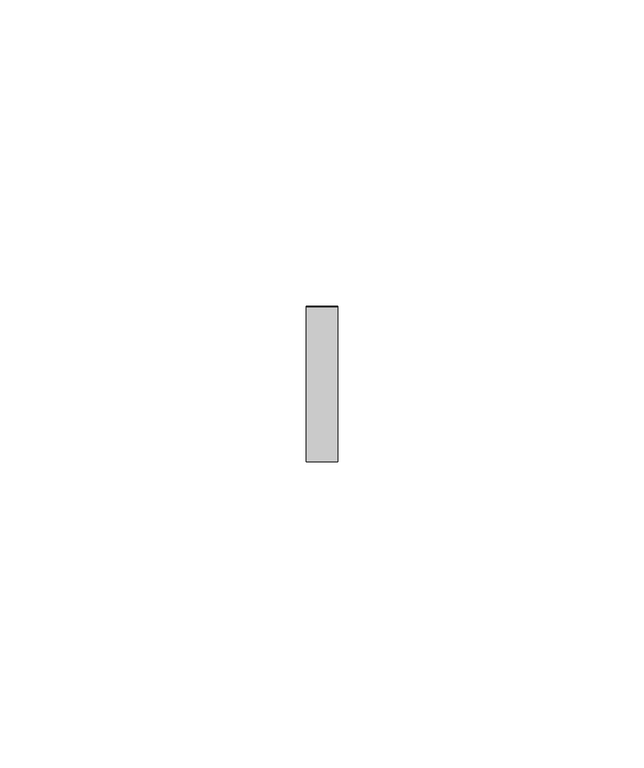
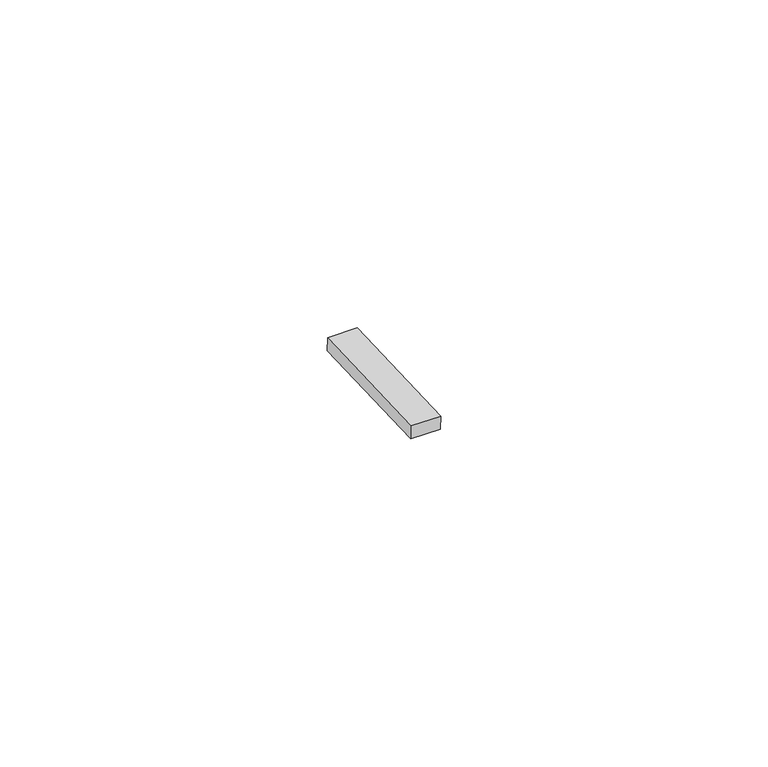
"""IFC4 building model written with IfcOpenShell, lengths in millimetres: proxy geometry, Inner panel:Inner panel:1:Inner panel:1 : Inner panel:Inner panel:300324:2:Inner panel:1:Inner panel:1 : Inner panel:Inner panel:300324:2 : Inner panel:Inner panel:1:Inner panel:1 : Inner panel:Inner panel:300324:300043:118 : Inner panel:Inner panel:1:Inner panel:1 : Inner panel:Inner panel:300324:2:Inner panel:1:Inner panel:1 : Inner panel:Inner panel:300324:2 : Inner panel:Inner panel:1:Inner panel:1 : Inner panel:Inner panel:300324:300043:308120."""

from ifc_helpers import new_model, si_unit, frame, origin, place, context, project, spatial, polyline, outline, extrude, source, transform, mapped, element, save


def generic_models_1f06ace7(model_context):
    return source(origin(), model_context, "Body", "SweptSolid", [
        extrude(outline(polyline([(0.0, -25.3999999), (0.0, 0.0), (5.2138089, 0.0), (5.2138089, -25.3999999), (0.0, -25.3999999)])), frame((593123.795117, -578962.7476805, 3951.4793391), z_axis=(0.0, -0.041630544712223896, 0.9991330730923502), x_axis=(-1.0, 0.0, 0.0)), (0.0, 0.0, 1.0), 2.4763745),
    ])


if __name__ == "__main__":
    model = new_model("IFC4")
    model_context = context("Model", 3, world=origin())
    ifc_project = project(units=[si_unit("LENGTHUNIT", "METRE", prefix="MILLI")], contexts=[model_context])
    site = spatial("IfcSite", under=ifc_project)
    building = spatial("IfcBuilding", under=site)
    placement = place(None, origin())
    generic_models_shape = generic_models_1f06ace7(model_context)
    element("IfcBuildingElementProxy", 1, Name="Inner panel:Inner panel:1:Inner panel:1 : Inner panel:Inner panel:300324:2:Inner panel:1:Inner panel:1 : Inner panel:Inner panel:300324:2 : Inner panel:Inner panel:1:Inner panel:1 : Inner panel:Inner panel:300324:300043:118 : Inner panel:Inner panel:1:Inner panel:1 : Inner panel:Inner panel:300324:2:Inner panel:1:Inner panel:1 : Inner panel:Inner panel:300324:2 : Inner panel:Inner panel:1:Inner panel:1 : Inner panel:Inner panel:300324:300043:308120", ObjectType="Inner panel:Inner panel:1:Inner panel:1 : Inner panel:Inner panel:300324:2:Inner panel:1:Inner panel:1 : Inner panel:Inner panel:300324:2 : Inner panel:Inner panel:1:Inner panel:1 : Inner panel:Inner panel:300324:300043:118 : Inner panel:Inner panel:1:Inner panel:1 : Inner panel:Inner panel:300324:2:Inner panel:1:Inner panel:1 : Inner panel:Inner panel:300324:2 : Inner panel:Inner panel:1:Inner panel:1 : Inner panel:Inner panel:300324:300043:308120", at=placement, inside=building, context=model_context, shape_type="MappedRepresentation", body=[
        mapped(generic_models_shape, transform((0.0, 0.0, 0.0), x_axis=(1.0, 0.0, 0.0), y_axis=(0.0, 1.0, 0.0), z_axis=(0.0, 0.0, 1.0))),
    ])
    save(model, "model.ifc")

# Revit data of these elements
# Type "Inner panel:Inner panel:1:Inner panel:1 : Inner panel:Inner panel:300324:2:Inner panel:1:Inner panel:1 : Inner panel:Inner panel:300324:2 : Inner panel:Inner panel:1:Inner panel:1 : Inner panel:Inner panel:300324:300043:118 : Inner panel:Inner panel:1:Inner panel:1 : Inner panel:Inner panel:300324:2:Inner panel:1:Inner panel:1 : Inner panel:Inner panel:300324:2 : Inner panel:Inner panel:1:Inner panel:1 : Inner panel:Inner panel:300324:300043:308120"
#   NameOverride = "Inner panel:Inner panel:1:Inner panel:1 : Inner panel:Inner panel:300324:2:Inner panel:1:Inner panel:1 : Inner panel:Inner panel:300324:2 : Inner panel:Inner panel:1:Inner panel:1 : Inner panel:Inner panel:300324:300043:308120"
#   ObjectTypeOverride = "Inner panel:1:Inner panel:1 : Inner panel:Inner panel:300324:2 : Inner panel:Inner panel:1:Inner panel:1 : Inner panel:Inner panel:300324:300043"
#   Reference = "Inner panel"
#   Tag = "308120"
# Element 1 (IfcBuildingElementProxy, "Inner panel:Inner panel:1:Inner panel:1 : Inner panel:Inner panel:300324:2:Inner panel:1:Inner panel:1 : Inner panel:Inner panel:300324:2 : Inner panel:Inner panel:1:Inner panel:1 : Inner panel:Inner panel:300324:300043:118 : Inner panel:Inner panel:1:Inner panel:1 : Inner panel:Inner panel:300324:2:Inner panel:1:Inner panel:1 : Inner panel:Inner panel:300324:2 : Inner panel:Inner panel:1:Inner panel:1 : Inner panel:Inner panel:300324:300043:308120")
#   Materials on its faces: "AT CLIP - 1\" WIDE NON ABSORBENT, WEATHER-RESISTANT NEOPRENE/EPDM/SBR FOAM"
# Materials
#   "AT CLIP - 1\" WIDE NON ABSORBENT, WEATHER-RESISTANT NEOPRENE/EPDM/SBR FOAM": class "Generic", colour RGB 85 85 85, transparency 0, Cost = 0
